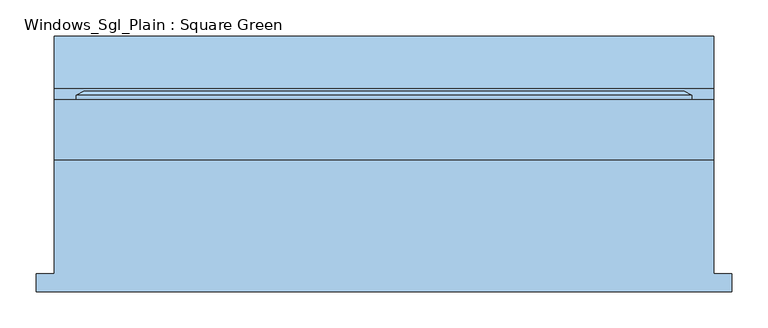
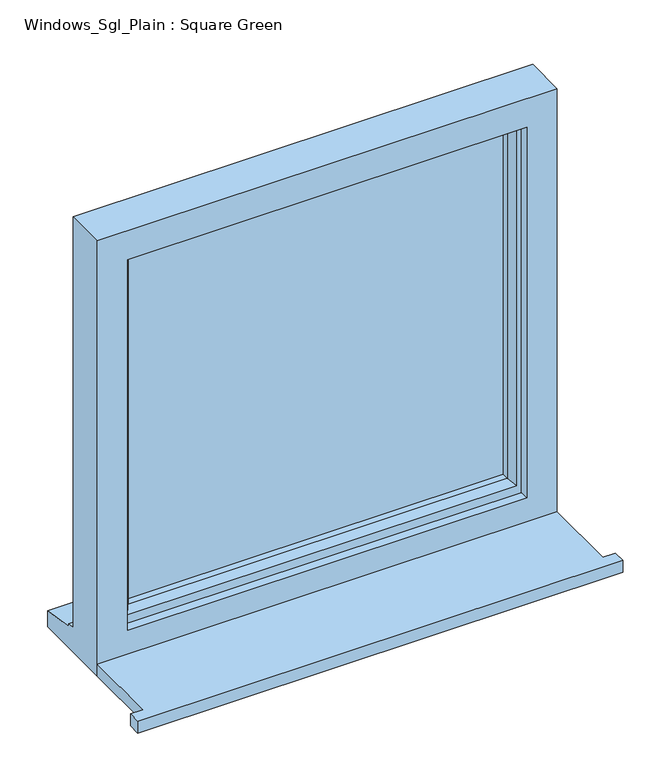
"""IFC4 building model written with IfcOpenShell, lengths in millimetres: window geometry, Windows_Sgl_Plain : Square Green."""

from ifc_helpers import new_model, si_unit, frame, origin, place, context, project, spatial, polyline, outline, extrude, faceted_brep, source, transform, mapped, element, save


def windows_sgl_plain_square_green_b9caa461(model_context):
    return source(origin(), model_context, "Body", "SolidModel", [
        extrude(outline(polyline([(-480.0, -161.5434322), (-480.0, -136.5434322), (-455.0, -136.5434322), (-455.0, 20.4565678), (455.0, 20.4565678), (455.0, -136.5434322), (480.0, -136.5434322), (480.0, -161.5434322), (-480.0, -161.5434322)])), frame((0.0, 0.0, 1200.0), z_axis=(0.0, 0.0, 1.0), x_axis=(1.0, 0.0, 0.0)), (0.0, 0.0, 1.0), 25.0),
        faceted_brep([(-455.0, 20.4565678, 1200.0), (455.0, 20.4565678, 1200.0), (455.0, 20.4565678, 2110.0), (-455.0, 20.4565678, 2110.0), (-395.0, 20.4565678, 2050.0), (395.0, 20.4565678, 2050.0), (395.0, 20.4565678, 1275.0), (-395.0, 20.4565678, 1275.0), (-455.0, 103.4565678, 2110.0), (-455.0, 103.4565678, 1251.0), (-455.0, 118.4565678, 1249.68767), (-455.0, 118.4565678, 1244.7449676), (-455.0, 190.9565678, 1233.8088847), (-455.0, 190.9565678, 1200.0), (455.0, 103.4565678, 2110.0), (455.0, 103.4565678, 1251.0), (-415.0, 103.4565678, 2070.0), (-415.0, 103.4565678, 1263.0), (415.0, 103.4565678, 1263.0), (415.0, 103.4565678, 2070.0), (-415.0, 38.4565678, 2070.0), (-415.0, 38.4565678, 1263.0), (415.0, 38.4565678, 2070.0), (415.0, 38.4565678, 1263.0), (-395.0, 38.4565678, 2050.0), (-395.0, 38.4565678, 1275.0), (395.0, 38.4565678, 1275.0), (395.0, 38.4565678, 2050.0), (455.0, 190.9565678, 1200.0), (455.0, 190.9565678, 1233.8088847), (455.0, 118.4565678, 1244.7449676), (455.0, 118.4565678, 1249.68767)], [[[0, 1, 2, 3], [4, 5, 6, 7]], [[0, 3, 8, 9, 10, 11, 12, 13]], [[9, 8, 14, 15], [16, 17, 18, 19]], [[17, 16, 20, 21]], [[20, 22, 23, 21], [24, 25, 26, 27]], [[24, 4, 7, 25]], [[3, 2, 14, 8]], [[16, 19, 22, 20]], [[5, 4, 24, 27]], [[15, 14, 2, 1, 28, 29, 30, 31]], [[19, 18, 23, 22]], [[5, 27, 26, 6]], [[28, 1, 0, 13]], [[29, 28, 13, 12]], [[30, 29, 12, 11]], [[31, 30, 11, 10]], [[15, 31, 10, 9]], [[21, 23, 18, 17]], [[7, 6, 26, 25]]]),
        extrude(outline(polyline([(385.0, 67.4565678), (-385.0, 67.4565678), (-385.0, 91.4565678), (385.0, 91.4565678), (385.0, 67.4565678)])), frame((0.0, 0.0, 1293.0), z_axis=(0.0, 0.0, 1.0), x_axis=(1.0, 0.0, 0.0)), (0.0, 0.0, 1.0), 747.0),
        faceted_brep([(-425.0, 103.4565678, 2080.0), (-425.0, 109.2300705, 2080.0), (-425.0, 109.2300705, 1253.0), (-425.0, 103.4565678, 1253.0), (-415.0, 38.4565678, 2070.0), (-415.0, 103.4565678, 2070.0), (-415.0, 103.4565678, 1263.0), (-415.0, 38.4565678, 1263.0), (-375.0, 52.9494677, 2030.0), (-385.1480377, 38.4565678, 2040.1480377), (-385.1480377, 38.4565678, 1292.8519623), (-375.0, 52.9494677, 1303.0), (-375.0, 67.4565678, 2030.0), (-375.0, 67.4565678, 1303.0), (-385.0, 91.4565678, 2040.0), (-385.0, 67.4565678, 2040.0), (-385.0, 67.4565678, 1293.0), (-385.0, 91.4565678, 1293.0), (-375.0, 109.2300705, 2030.0), (-375.0, 91.4565678, 2030.0), (-375.0, 91.4565678, 1303.0), (-375.0, 109.2300705, 1303.0), (-392.4457548, 115.0035732, 2047.4457548), (-392.4457548, 115.0035732, 1285.5542452), (-414.2153903, 115.0035732, 2069.2153903), (-414.2153903, 115.0035732, 1263.7846097), (425.0, 109.2300705, 1253.0), (425.0, 103.4565678, 1253.0), (415.0, 103.4565678, 1263.0), (415.0, 38.4565678, 1263.0), (385.1480377, 38.4565678, 1292.8519623), (375.0, 52.9494677, 1303.0), (375.0, 67.4565678, 1303.0), (385.0, 67.4565678, 1293.0), (385.0, 91.4565678, 1293.0), (375.0, 91.4565678, 1303.0), (375.0, 109.2300705, 1303.0), (392.4457548, 115.0035732, 1285.5542452), (414.2153903, 115.0035732, 1263.7846097), (425.0, 109.2300705, 2080.0), (425.0, 103.4565678, 2080.0), (415.0, 103.4565678, 2070.0), (415.0, 38.4565678, 2070.0), (385.1480377, 38.4565678, 2040.1480377), (375.0, 52.9494677, 2030.0), (375.0, 67.4565678, 2030.0), (385.0, 67.4565678, 2040.0), (385.0, 91.4565678, 2040.0), (375.0, 91.4565678, 2030.0), (375.0, 109.2300705, 2030.0), (392.4457548, 115.0035732, 2047.4457548), (414.2153903, 115.0035732, 2069.2153903)], [[[0, 1, 2, 3]], [[4, 5, 6, 7]], [[8, 9, 10, 11]], [[12, 8, 11, 13]], [[14, 15, 16, 17]], [[18, 19, 20, 21]], [[22, 18, 21, 23]], [[1, 24, 25, 2]], [[3, 2, 26, 27]], [[7, 6, 28, 29]], [[11, 10, 30, 31]], [[13, 11, 31, 32]], [[17, 16, 33, 34]], [[21, 20, 35, 36]], [[23, 21, 36, 37]], [[2, 25, 38, 26]], [[27, 26, 39, 40]], [[29, 28, 41, 42]], [[31, 30, 43, 44]], [[32, 31, 44, 45]], [[34, 33, 46, 47]], [[36, 35, 48, 49]], [[37, 36, 49, 50]], [[26, 38, 51, 39]], [[40, 39, 1, 0]], [[3, 27, 40, 0], [5, 41, 28, 6]], [[42, 41, 5, 4]], [[7, 29, 42, 4], [9, 43, 30, 10]], [[44, 43, 9, 8]], [[45, 44, 8, 12]], [[15, 46, 33, 16], [13, 32, 45, 12]], [[47, 46, 15, 14]], [[17, 34, 47, 14], [19, 48, 35, 20]], [[49, 48, 19, 18]], [[50, 49, 18, 22]], [[24, 51, 38, 25], [23, 37, 50, 22]], [[39, 51, 24, 1]]]),
    ])


if __name__ == "__main__":
    model = new_model("IFC4")
    model_context = context("Model", 3, world=origin())
    ifc_project = project(units=[si_unit("LENGTHUNIT", "METRE", prefix="MILLI")], contexts=[model_context])
    site = spatial("IfcSite", under=ifc_project)
    building = spatial("IfcBuilding", under=site)
    placement = place(None, origin())
    windows_sgl_plain_square_green_shape = windows_sgl_plain_square_green_b9caa461(model_context)
    element("IfcWindow", 1, ObjectType="Windows_Sgl_Plain : Square Green", at=placement, inside=building, context=model_context, shape_type="MappedRepresentation", body=[
        mapped(windows_sgl_plain_square_green_shape, transform((0.0, 0.0, 0.0), x_axis=(1.0, 0.0, 0.0), y_axis=(0.0, 1.0, 0.0), z_axis=(0.0, 0.0, 1.0))),
    ])
    save(model, "model.ifc")

# Revit data of these elements
# Type "Windows_Sgl_Plain : Square Green"
#   Type Mark = "51"
#   Operation = "SinglePanel"
#   Construction Type Id = "SGL"
#   Manufacturer = "Revit"
#   Keynote = "L10"
#   Analytic Construction = "Large single-glazed windows"
#   Wrap Layers (Ext) from Ext = 102.5 mm
#   Wrap Layers (Int) from Ext = 177.5 mm
#   Window Board Projection = 25 mm
#   Window Board Extension = 25 mm
#   Visual Light Transmittance = 0.9
#   Solar Heat Gain Coefficient = 0.86
#   Rough Width = 910 mm
#   Rough Height = 910 mm
#   Height = 910 mm
#   Width = 910 mm
#   Heat Transfer Coefficient (U) = 5.5617 W/(m²·K)
#   Glazing Thickness = 24 mm
#   FrameOffset - External = 50 mm
#   Frame Depth = 65 mm
#   Default Head Height = 2110 mm
#   Cill Depth = 87.5 mm
#   Cavity Closer Width = 50 mm
#   Cavity Closer Offset from Ext = 102.5 mm
#   Cavity Closer Depth = 85 mm
#   Vis - Cavity Closers = yes
#   Material Trim = Window Frame
#   Material Glass = Green Glass
#   Material Frame = Window Frame
#   Wall Closure = (empty or 0)
# Element 1 (IfcWindow, "Windows_Sgl_Plain : Square Green")
#   Materials on its faces: "Window Frame", "Green Glass"
# Materials
#   "Window Frame": class "Miscellaneous", colour RGB 249 249 249, transparency 0, Keynote = "L10", Cost = 0
#   "Green Glass": class "Glass", colour RGB 0 242 0, transparency 0.8, Description = "Soda Lime Glass", Cost = 0
